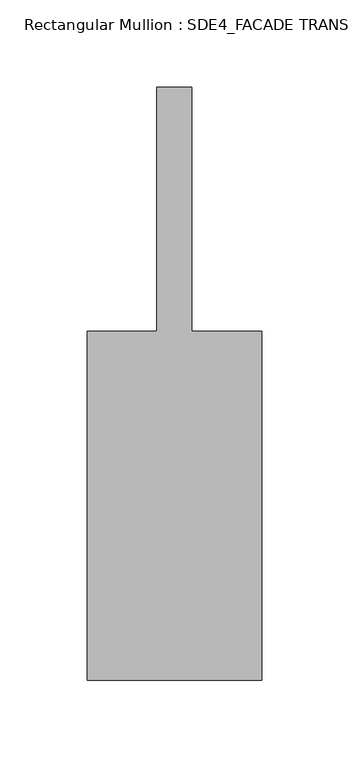
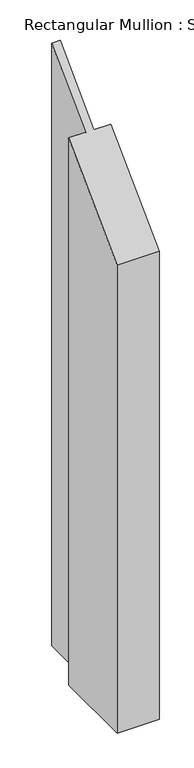
"""IFC4 building model written with IfcOpenShell, lengths in millimetres: member geometry, Rectangular Mullion : SDE4_FACADE TRANSOM TYPE 1."""

from ifc_helpers import new_model, si_unit, origin, place, context, project, spatial, faceted_brep, source, transform, mapped, element, save


def rectangular_mullion_sde4_facade_transom_type_1_ef13bfed(model_context):
    return source(origin(), model_context, "Body", "Brep", [
        faceted_brep([(50.0, -132.5, -1312.8649957), (-50.0, -132.5, -1312.8649957), (-50.0, 67.5, -1312.8649957), (-10.0, 67.5, -1312.8649957), (-10.0, 207.5, -1312.8649957), (10.0, 207.5, -1312.8649957), (10.0, 67.5, -1312.8649957), (50.0, 67.5, -1312.8649957), (50.0, 67.5, 67.5), (50.0, -132.5, -132.5), (10.0, 67.5, 67.5), (10.0, 207.5, 207.5), (-10.0, 207.5, 207.5), (-10.0, 67.5, 67.5), (-50.0, 67.5, 67.5), (-50.0, -132.5, -132.5)], [[[0, 1, 2, 3, 4, 5, 6, 7]], [[8, 9, 0, 7]], [[10, 8, 7, 6]], [[11, 10, 6, 5]], [[12, 11, 5, 4]], [[13, 12, 4, 3]], [[14, 13, 3, 2]], [[15, 14, 2, 1]], [[9, 15, 1, 0]], [[9, 8, 10, 11, 12, 13, 14, 15]]]),
    ])


if __name__ == "__main__":
    model = new_model("IFC4")
    model_context = context("Model", 3, world=origin())
    ifc_project = project(units=[si_unit("LENGTHUNIT", "METRE", prefix="MILLI")], contexts=[model_context])
    site = spatial("IfcSite", under=ifc_project)
    building = spatial("IfcBuilding", under=site)
    placement = place(None, origin())
    rectangular_mullion_sde4_facade_transom_type_1_shape = rectangular_mullion_sde4_facade_transom_type_1_ef13bfed(model_context)
    element("IfcMember", 1, ObjectType="Rectangular Mullion : SDE4_FACADE TRANSOM TYPE 1", at=placement, inside=building, context=model_context, shape_type="MappedRepresentation", body=[
        mapped(rectangular_mullion_sde4_facade_transom_type_1_shape, transform((0.0, 0.0, 0.0), x_axis=(1.0, 0.0, 0.0), y_axis=(0.0, 1.0, 0.0), z_axis=(0.0, 0.0, 1.0))),
    ])
    save(model, "model.ifc")

# Revit data of these elements
# Type "Rectangular Mullion : SDE4_FACADE TRANSOM TYPE 1"
#   built-in parameter 1007322 = 1.11549 (stored number, unit not read)
#   built-in parameter 1007321 = 0.164042 (stored number, unit not read)
#   built-in parameter 1007320 = 0.164042 (stored number, unit not read)
